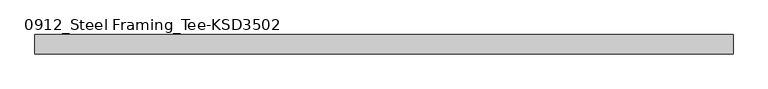
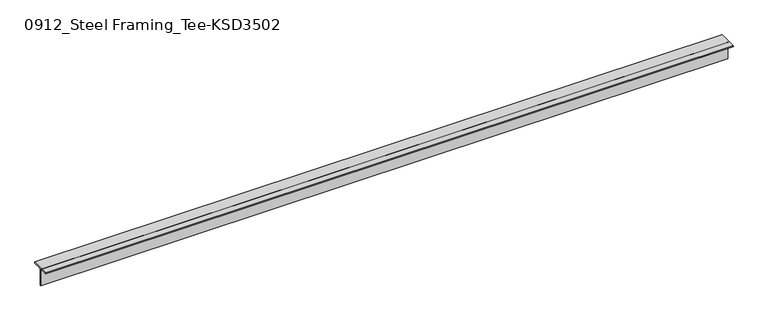
"""IFC4 building model written with IfcOpenShell, lengths in millimetres: member geometry, 0912_Steel Framing_Tee-KSD3502 : H_SB_ASB_CT-150x150x6.5x9."""

from ifc_helpers import new_model, si_unit, point, frame, frame_2d, origin, place, context, project, spatial, polyline, circle_curve, trimmed, segment, composite_curve, outline, extrude, source, transform, mapped, element, save


def member_0912_steel_framing_tee_ksd3502_e24d29f6(model_context):
    return source(origin(), model_context, "Body", "SweptSolid", [
        extrude(outline(composite_curve([segment(polyline([(-75.0, 75.0), (75.0, 75.0), (75.0, 66.0), (16.25, 66.0)]), True, "CONTINUOUS"), segment(trimmed(circle_curve(frame_2d((16.25, 53.0)), 13.0), [point((16.25, 66.0))], [point((3.25, 53.0))], True, "CARTESIAN"), True, "CONTINUOUS"), segment(polyline([(3.25, 53.0), (3.25, -75.0), (-3.25, -75.0), (-3.25, 53.0)]), True, "CONTINUOUS"), segment(trimmed(circle_curve(frame_2d((-16.25, 53.0)), 13.0), [point((-3.25, 53.0))], [point((-16.25, 66.0))], True, "CARTESIAN"), True, "CONTINUOUS"), segment(polyline([(-16.25, 66.0), (-75.0, 66.0), (-75.0, 75.0)]), True, "CONTINUOUS")], self_intersect=False)), frame((-2674.75, 0.0, 0.0), z_axis=(1.0, 0.0, 0.0), x_axis=(0.0, 1.0, 0.0)), (0.0, 0.0, 1.0), 5417.7),
    ])


if __name__ == "__main__":
    model = new_model("IFC4")
    model_context = context("Model", 3, world=origin())
    ifc_project = project(units=[si_unit("LENGTHUNIT", "METRE", prefix="MILLI")], contexts=[model_context])
    site = spatial("IfcSite", under=ifc_project)
    building = spatial("IfcBuilding", under=site)
    placement = place(None, origin())
    member_0912_steel_framing_tee_ksd3502_shape = member_0912_steel_framing_tee_ksd3502_e24d29f6(model_context)
    element("IfcMember", 1, ObjectType="0912_Steel Framing_Tee-KSD3502 : H_SB_ASB_CT-150x150x6.5x9", at=placement, inside=building, context=model_context, shape_type="MappedRepresentation", body=[
        mapped(member_0912_steel_framing_tee_ksd3502_shape, transform((0.0, 0.0, 0.0), x_axis=(1.0, 0.0, 0.0), y_axis=(0.0, 1.0, 0.0), z_axis=(0.0, 0.0, 1.0))),
    ])
    save(model, "model.ifc")

# Revit data of these elements
# Type "0912_Steel Framing_Tee-KSD3502 : H_SB_ASB_CT-150x150x6.5x9"
#   H_WM Code_1 = "S01AA003-00001 | Main Steel Structure Fabrication Work | Shelter/Building | Light Steel - Standard (30KG/M>Weight) | Material: (   )"
#   H_WM Code_2 = "S03AA029-00001 | Main Steel Structure Erection Work | Shelter/Building | Light Steel (30KG/M>Weight) | Material: (   )"
#   H_WM Code_3 = "S01AA010-00001 | Main Steel Structure Fabrication Work | Shelter/Building | Steel Painting/Coating | for Non-Fireproofed Steel Surface, Surface Preparation, Primer, Second & Final Coat | Material: (   )"
#   H_Q'ty Cal Type Tag = "SB-Q2"
#   Width = 15.0 cm
#   Web Thickness = 0.65 cm
#   Web Fillet = 1.3 cm
#   Section Area = 23.39 cm²
#   Perimeter = 0.60 m²/m
#   Nominal Weight = 18.40 kgf/m
#   Height = 15.0 cm
#   Flange Thickness = 0.9 cm
#   Centroid Vertical = 7.5 cm
#   Centroid Horizontal = 7.5 cm
#   Length [instance default] = 1.5000 m
#   Structural Material [instance default] = Steel, 45-345
#   Warping Constant = (empty or 0)
#   Torsional Moment of Inertia = 0
#   Section Name Key = ""
#   Plastic Modulus weak axis = 0
#   Plastic Modulus strong axis = 0
#   Moment of Inertia weak axis = 0
#   Moment of Inertia strong axis = 0
#   Elastic Modulus weak axis = 0
#   Elastic Modulus strong axis = 0
#   Bolt Spacing = 0
#   Assembly Code = ""
# Element 1 (IfcMember, "0912_Steel Framing_Tee-KSD3502 : H_SB_ASB_CT-150x150x6.5x9")
#   Structural Material = none
# Materials
#   "Steel, 45-345": class "Metal", colour RGB 189 187 185, transparency 0, Description = "Steel 345 MPa", Cost = 0
